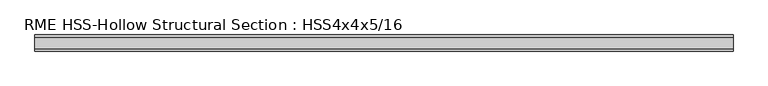
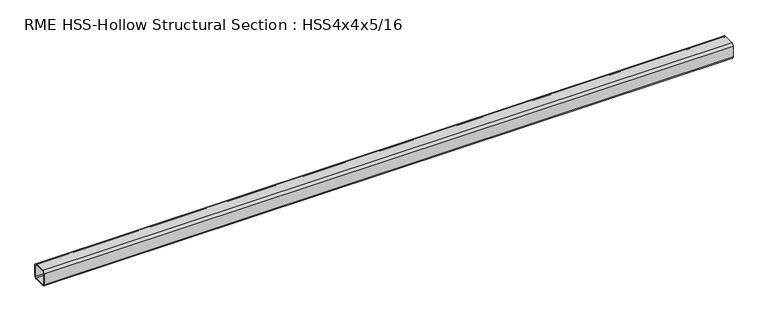
"""IFC4 building model written with IfcOpenShell, lengths in millimetres: member geometry, RME HSS-Hollow Structural Section : HSS4x4x5/16."""

from ifc_helpers import new_model, si_unit, point, frame, frame_2d, origin, place, context, project, spatial, polyline, circle_curve, trimmed, segment, composite_curve, outline, extrude, source, transform, mapped, element, save


def rme_hss_hollow_structural_section_hss4x4x5_16_7e9617a0(model_context):
    return source(origin(), model_context, "Body", "SweptSolid", [
        extrude(outline(composite_curve([segment(polyline([(50.8, 36.0172), (50.8, -36.0172)]), True, "CONTINUOUS"), segment(trimmed(circle_curve(frame_2d((36.0172, -36.0172)), 14.7828), [point((50.8, -36.0172))], [point((36.0172, -50.8))], False, "CARTESIAN"), True, "CONTINUOUS"), segment(polyline([(36.0172, -50.8), (-36.0172, -50.8)]), True, "CONTINUOUS"), segment(trimmed(circle_curve(frame_2d((-36.0172, -36.0172)), 14.7828), [point((-36.0172, -50.8))], [point((-50.8, -36.0172))], False, "CARTESIAN"), True, "CONTINUOUS"), segment(polyline([(-50.8, -36.0172), (-50.8, 36.0172)]), True, "CONTINUOUS"), segment(trimmed(circle_curve(frame_2d((-36.0172, 36.0172)), 14.7828), [point((-50.8, 36.0172))], [point((-36.0172, 50.8))], False, "CARTESIAN"), True, "CONTINUOUS"), segment(polyline([(-36.0172, 50.8), (36.0172, 50.8)]), True, "CONTINUOUS"), segment(trimmed(circle_curve(frame_2d((36.0172, 36.0172)), 14.7828), [point((36.0172, 50.8))], [point((50.8, 36.0172))], False, "CARTESIAN"), True, "CONTINUOUS")], self_intersect=False), holes=[composite_curve([segment(trimmed(circle_curve(frame_2d((-36.0172, 36.0172)), 7.3914), [point((-36.0172, 43.4086))], [point((-43.4086, 36.0172))], True, "CARTESIAN"), True, "CONTINUOUS"), segment(polyline([(-43.4086, 36.0172), (-43.4086, -36.0172)]), True, "CONTINUOUS"), segment(trimmed(circle_curve(frame_2d((-36.0172, -36.0172)), 7.3914), [point((-43.4086, -36.0172))], [point((-36.0172, -43.4086))], True, "CARTESIAN"), True, "CONTINUOUS"), segment(polyline([(-36.0172, -43.4086), (36.0172, -43.4086)]), True, "CONTINUOUS"), segment(trimmed(circle_curve(frame_2d((36.0172, -36.0172)), 7.3914), [point((36.0172, -43.4086))], [point((43.4086, -36.0172))], True, "CARTESIAN"), True, "CONTINUOUS"), segment(polyline([(43.4086, -36.0172), (43.4086, 36.0172)]), True, "CONTINUOUS"), segment(trimmed(circle_curve(frame_2d((36.0172, 36.0172)), 7.3914), [point((43.4086, 36.0172))], [point((36.0172, 43.4086))], True, "CARTESIAN"), True, "CONTINUOUS"), segment(polyline([(36.0172, 43.4086), (-36.0172, 43.4086)]), True, "CONTINUOUS")], self_intersect=False)]), frame((-2362.5026588, 0.0, 0.0), z_axis=(1.0, 0.0, 0.0), x_axis=(0.0, 1.0, 0.0)), (0.0, 0.0, 1.0), 4407.147463),
    ])


if __name__ == "__main__":
    model = new_model("IFC4")
    model_context = context("Model", 3, world=origin())
    ifc_project = project(units=[si_unit("LENGTHUNIT", "METRE", prefix="MILLI")], contexts=[model_context])
    site = spatial("IfcSite", under=ifc_project)
    building = spatial("IfcBuilding", under=site)
    placement = place(None, origin())
    rme_hss_hollow_structural_section_hss4x4x5_16_shape = rme_hss_hollow_structural_section_hss4x4x5_16_7e9617a0(model_context)
    element("IfcMember", 1, ObjectType="RME HSS-Hollow Structural Section : HSS4x4x5/16", at=placement, inside=building, context=model_context, shape_type="MappedRepresentation", body=[
        mapped(rme_hss_hollow_structural_section_hss4x4x5_16_shape, transform((0.0, 0.0, 0.0), x_axis=(1.0, 0.0, 0.0), y_axis=(0.0, 1.0, 0.0), z_axis=(0.0, 0.0, 1.0))),
    ])
    save(model, "model.ifc")

# Revit data of these elements
# Type "RME HSS-Hollow Structural Section : HSS4x4x5/16"
#   Nominal Size = "HSS6x4"
#   Assembly Code = "B10"
#   Shape = "Square"
#   W = 14.8
#   Start Extension Calculation [instance default] = 10' - 0"
#   Start Extension [instance default] = -0' - 0 1/2"
#   End Extension Calculation [instance default] = 10' - 0"
#   End Extension [instance default] = -0' - 0 1/2"
#   Ht = 0' - 4"
#   Length [instance default] = 5' - 0"
#   b = 0' - 4"
#   kr = 0' - 0.582"
#   t = 0' - 0.291"
#   A = 0.0284722 SF
#   Structural Material [instance default] = Metal - Steel - ASTM A500 - Grade B - Rectangular and Square
# Element 1 (IfcMember, "RME HSS-Hollow Structural Section : HSS4x4x5/16")
#   Structural Material = Metal - Steel - ASTM A992
#   Materials on its faces: "Metal - Steel - ASTM A992"
# Materials
#   "Metal - Steel - ASTM A500 - Grade B - Rectangular and Square": class "Metal", colour RGB 255 128 0, transparency 0
#   "Metal - Steel - ASTM A992": class "Metal", colour RGB 255 128 0, transparency 0
